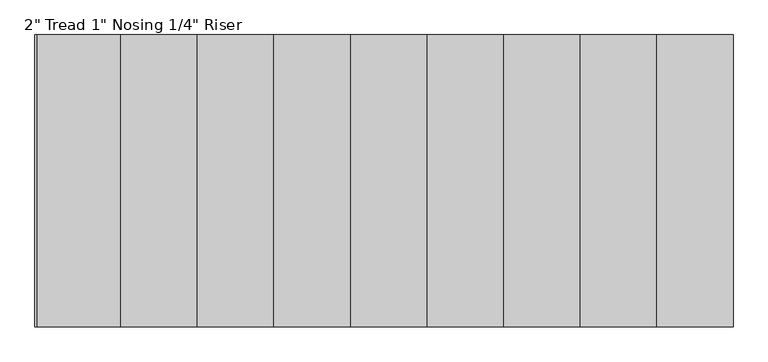
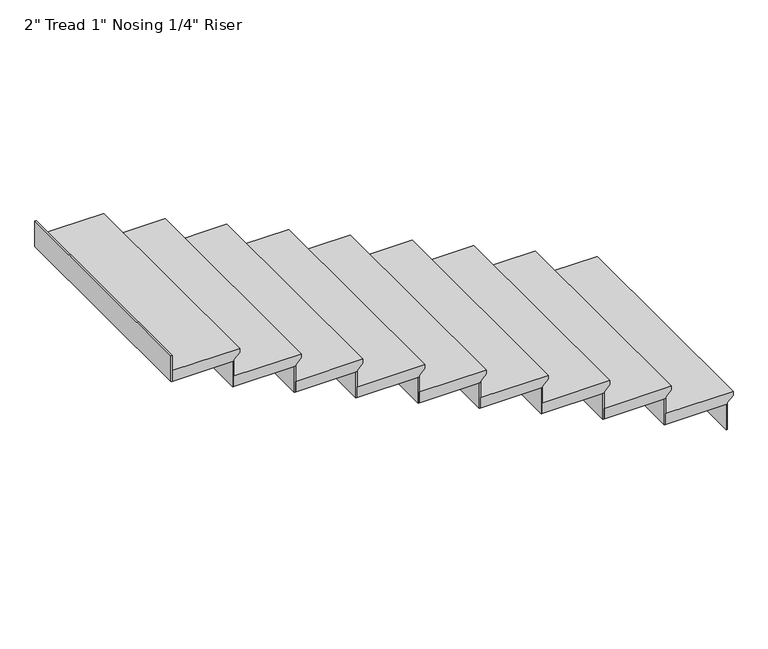
"""IFC4 building model written with IfcOpenShell, lengths in millimetres: stair flight geometry."""

from ifc_helpers import new_model, si_unit, frame, origin, place, context, project, spatial, polyline, outline, extrude, source, transform, mapped, element, save


def stair_flight_c64577be(model_context):
    return source(origin(), model_context, "Body", "SweptSolid", [
        extrude(outline(polyline([(3459.8918919, 665956.388677), (3459.8918919, 665651.588677), (3409.0918919, 665651.588677), (3409.0918919, 665930.988677), (3415.4418919, 665930.988677), (3440.8418919, 665956.388677), (3459.8918919, 665956.388677)])), frame((0.0, -550482.8413841, 0.0), z_axis=(0.0, 1.0, 0.0), x_axis=(0.0, 0.0, 1.0)), (0.0, 0.0, 1.0), 1066.8),
        extrude(outline(polyline([(665924.638677, -549416.0413841), (665930.988677, -549416.0413841), (665930.988677, -550482.8413841), (665924.638677, -550482.8413841), (665924.638677, -549416.0413841)])), frame((0.0, 0.0, 3285.5243243), z_axis=(0.0, 0.0, 1.0), x_axis=(1.0, 0.0, 0.0)), (0.0, 0.0, 1.0), 123.5675676),
        extrude(outline(polyline([(665645.238677, -549416.0413841), (665651.588677, -549416.0413841), (665651.588677, -550482.8413841), (665645.238677, -550482.8413841), (665645.238677, -549416.0413841)])), frame((0.0, 0.0, 3409.0918919), z_axis=(0.0, 0.0, 1.0), x_axis=(1.0, 0.0, 0.0)), (0.0, 0.0, 1.0), 123.5675676),
        extrude(outline(polyline([(3583.4594595, 665676.988677), (3583.4594595, 665372.188677), (3532.6594595, 665372.188677), (3532.6594595, 665651.588677), (3539.0094595, 665651.588677), (3564.4094595, 665676.988677), (3583.4594595, 665676.988677)])), frame((0.0, -550482.8413841, 0.0), z_axis=(0.0, 1.0, 0.0), x_axis=(0.0, 0.0, 1.0)), (0.0, 0.0, 1.0), 1066.8),
        extrude(outline(polyline([(665365.838677, -549416.0413841), (665372.188677, -549416.0413841), (665372.188677, -550482.8413841), (665365.838677, -550482.8413841), (665365.838677, -549416.0413841)])), frame((0.0, 0.0, 3532.6594595), z_axis=(0.0, 0.0, 1.0), x_axis=(1.0, 0.0, 0.0)), (0.0, 0.0, 1.0), 123.5675676),
        extrude(outline(polyline([(3707.027027, 665397.588677), (3707.027027, 665092.788677), (3656.227027, 665092.788677), (3656.227027, 665372.188677), (3662.577027, 665372.188677), (3687.977027, 665397.588677), (3707.027027, 665397.588677)])), frame((0.0, -550482.8413841, 0.0), z_axis=(0.0, 1.0, 0.0), x_axis=(0.0, 0.0, 1.0)), (0.0, 0.0, 1.0), 1066.8),
        extrude(outline(polyline([(665086.438677, -549416.0413841), (665092.788677, -549416.0413841), (665092.788677, -550482.8413841), (665086.438677, -550482.8413841), (665086.438677, -549416.0413841)])), frame((0.0, 0.0, 3656.227027), z_axis=(0.0, 0.0, 1.0), x_axis=(1.0, 0.0, 0.0)), (0.0, 0.0, 1.0), 123.5675676),
        extrude(outline(polyline([(3830.5945946, 665118.188677), (3830.5945946, 664813.388677), (3779.7945946, 664813.388677), (3779.7945946, 665092.788677), (3786.1445946, 665092.788677), (3811.5445946, 665118.188677), (3830.5945946, 665118.188677)])), frame((0.0, -550482.8413841, 0.0), z_axis=(0.0, 1.0, 0.0), x_axis=(0.0, 0.0, 1.0)), (0.0, 0.0, 1.0), 1066.8),
        extrude(outline(polyline([(664807.038677, -549416.0413841), (664813.388677, -549416.0413841), (664813.388677, -550482.8413841), (664807.038677, -550482.8413841), (664807.038677, -549416.0413841)])), frame((0.0, 0.0, 3779.7945946), z_axis=(0.0, 0.0, 1.0), x_axis=(1.0, 0.0, 0.0)), (0.0, 0.0, 1.0), 123.5675676),
        extrude(outline(polyline([(3954.1621622, 664838.788677), (3954.1621622, 664533.988677), (3903.3621622, 664533.988677), (3903.3621622, 664813.388677), (3909.7121622, 664813.388677), (3935.1121622, 664838.788677), (3954.1621622, 664838.788677)])), frame((0.0, -550482.8413841, 0.0), z_axis=(0.0, 1.0, 0.0), x_axis=(0.0, 0.0, 1.0)), (0.0, 0.0, 1.0), 1066.8),
        extrude(outline(polyline([(664527.638677, -549416.0413841), (664533.988677, -549416.0413841), (664533.988677, -550482.8413841), (664527.638677, -550482.8413841), (664527.638677, -549416.0413841)])), frame((0.0, 0.0, 3903.3621622), z_axis=(0.0, 0.0, 1.0), x_axis=(1.0, 0.0, 0.0)), (0.0, 0.0, 1.0), 123.5675676),
        extrude(outline(polyline([(4077.7297297, 664559.388677), (4077.7297297, 664254.588677), (4026.9297297, 664254.588677), (4026.9297297, 664533.988677), (4033.2797297, 664533.988677), (4058.6797297, 664559.388677), (4077.7297297, 664559.388677)])), frame((0.0, -550482.8413841, 0.0), z_axis=(0.0, 1.0, 0.0), x_axis=(0.0, 0.0, 1.0)), (0.0, 0.0, 1.0), 1066.8),
        extrude(outline(polyline([(664248.238677, -549416.0413841), (664254.588677, -549416.0413841), (664254.588677, -550482.8413841), (664248.238677, -550482.8413841), (664248.238677, -549416.0413841)])), frame((0.0, 0.0, 4026.9297297), z_axis=(0.0, 0.0, 1.0), x_axis=(1.0, 0.0, 0.0)), (0.0, 0.0, 1.0), 123.5675676),
        extrude(outline(polyline([(4201.2972973, 664279.988677), (4201.2972973, 663975.188677), (4150.4972973, 663975.188677), (4150.4972973, 664254.588677), (4156.8472973, 664254.588677), (4182.2472973, 664279.988677), (4201.2972973, 664279.988677)])), frame((0.0, -550482.8413841, 0.0), z_axis=(0.0, 1.0, 0.0), x_axis=(0.0, 0.0, 1.0)), (0.0, 0.0, 1.0), 1066.8),
        extrude(outline(polyline([(663968.838677, -549416.0413841), (663975.188677, -549416.0413841), (663975.188677, -550482.8413841), (663968.838677, -550482.8413841), (663968.838677, -549416.0413841)])), frame((0.0, 0.0, 4150.4972973), z_axis=(0.0, 0.0, 1.0), x_axis=(1.0, 0.0, 0.0)), (0.0, 0.0, 1.0), 123.5675676),
        extrude(outline(polyline([(4324.8648649, 664000.588677), (4324.8648649, 663695.788677), (4274.0648649, 663695.788677), (4274.0648649, 663975.188677), (4280.4148649, 663975.188677), (4305.8148649, 664000.588677), (4324.8648649, 664000.588677)])), frame((0.0, -550482.8413841, 0.0), z_axis=(0.0, 1.0, 0.0), x_axis=(0.0, 0.0, 1.0)), (0.0, 0.0, 1.0), 1066.8),
        extrude(outline(polyline([(663689.438677, -549416.0413841), (663695.788677, -549416.0413841), (663695.788677, -550482.8413841), (663689.438677, -550482.8413841), (663689.438677, -549416.0413841)])), frame((0.0, 0.0, 4274.0648649), z_axis=(0.0, 0.0, 1.0), x_axis=(1.0, 0.0, 0.0)), (0.0, 0.0, 1.0), 123.5675676),
        extrude(outline(polyline([(663410.038677, -549416.0413841), (663416.388677, -549416.0413841), (663416.388677, -550482.8413841), (663410.038677, -550482.8413841), (663410.038677, -549416.0413841)])), frame((0.0, 0.0, 4397.6324324), z_axis=(0.0, 0.0, 1.0), x_axis=(1.0, 0.0, 0.0)), (0.0, 0.0, 1.0), 123.5675676),
        extrude(outline(polyline([(4448.4324324, 663721.188677), (4448.4324324, 663416.388677), (4397.6324324, 663416.388677), (4397.6324324, 663695.788677), (4403.9824324, 663695.788677), (4429.3824324, 663721.188677), (4448.4324324, 663721.188677)])), frame((0.0, -550482.8413841, 0.0), z_axis=(0.0, 1.0, 0.0), x_axis=(0.0, 0.0, 1.0)), (0.0, 0.0, 1.0), 1066.8),
    ])


if __name__ == "__main__":
    model = new_model("IFC4")
    model_context = context("Model", 3, world=origin())
    ifc_project = project(units=[si_unit("LENGTHUNIT", "METRE", prefix="MILLI")], contexts=[model_context])
    site = spatial("IfcSite", under=ifc_project)
    building = spatial("IfcBuilding", under=site)
    placement = place(None, origin())
    stair_flight_shape = stair_flight_c64577be(model_context)
    element("IfcStairFlight", 1, ObjectType="2\" Tread 1\" Nosing 1/4\" Riser", at=placement, inside=building, context=model_context, shape_type="MappedRepresentation", body=[
        mapped(stair_flight_shape, transform((0.0, 0.0, 0.0), x_axis=(1.0, 0.0, 0.0), y_axis=(0.0, 1.0, 0.0), z_axis=(0.0, 0.0, 1.0))),
    ])
    save(model, "model.ifc")
